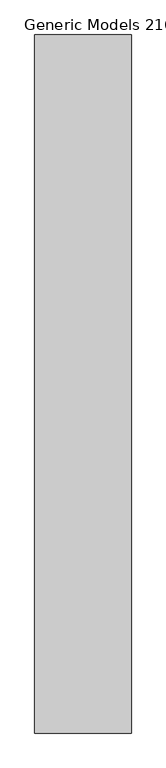
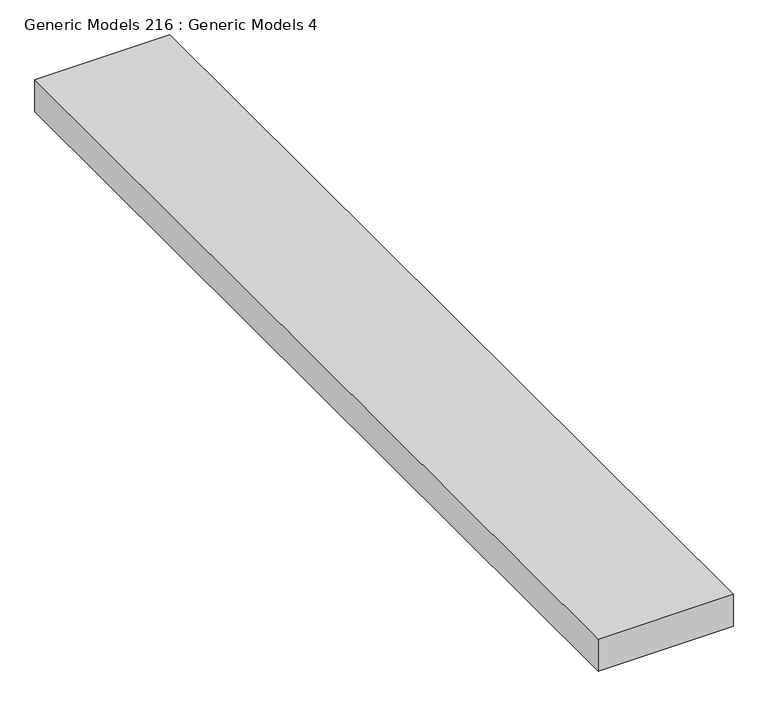
"""IFC4 building model written with IfcOpenShell, lengths in millimetres: proxy geometry, Generic Models 216 : Generic Models 4."""

from ifc_helpers import new_model, si_unit, frame, origin, place, context, project, spatial, polyline, outline, extrude, source, transform, mapped, element, save


def generic_models_216_generic_models_4_3b81cdab(model_context):
    return source(origin(), model_context, "Body", "SweptSolid", [
        extrude(outline(polyline([(-6661.9105076, -464.1230338), (-7702.282997, -464.1230338), (-7702.282997, 7054.2769662), (-6661.9105076, 7054.2769662), (-6661.9105076, -464.1230338)])), frame((0.0, 0.0, 126385.8816024), z_axis=(0.0, 0.0, 1.0), x_axis=(1.0, 0.0, 0.0)), (0.0, 0.0, 1.0), 260.35),
    ])


if __name__ == "__main__":
    model = new_model("IFC4")
    model_context = context("Model", 3, world=origin())
    ifc_project = project(units=[si_unit("LENGTHUNIT", "METRE", prefix="MILLI")], contexts=[model_context])
    site = spatial("IfcSite", under=ifc_project)
    building = spatial("IfcBuilding", under=site)
    placement = place(None, origin())
    generic_models_216_generic_models_4_shape = generic_models_216_generic_models_4_3b81cdab(model_context)
    element("IfcBuildingElementProxy", 1, Name="Generic Models 216 : Generic Models 4", ObjectType="Generic Models 216 : Generic Models 4", at=placement, inside=building, context=model_context, shape_type="MappedRepresentation", body=[
        mapped(generic_models_216_generic_models_4_shape, transform((0.0, 0.0, 0.0), x_axis=(1.0, 0.0, 0.0), y_axis=(0.0, 1.0, 0.0), z_axis=(0.0, 0.0, 1.0))),
    ])
    save(model, "model.ifc")

# Revit data of these elements
# Element 1 (IfcBuildingElementProxy, "Generic Models 216 : Generic Models 4")
#   Materials on its faces: "_BATT INSUL. (R-FACTOR = R38 MIN) OVER CLASS II VAPOR RETARDER(TOWARD INTERIOR)"
# Materials
#   "_BATT INSUL. (R-FACTOR = R38 MIN) OVER CLASS II VAPOR RETARDER(TOWARD INTERIOR)": class "Generic", colour RGB 200 166 247, transparency 0, Cost = 0
